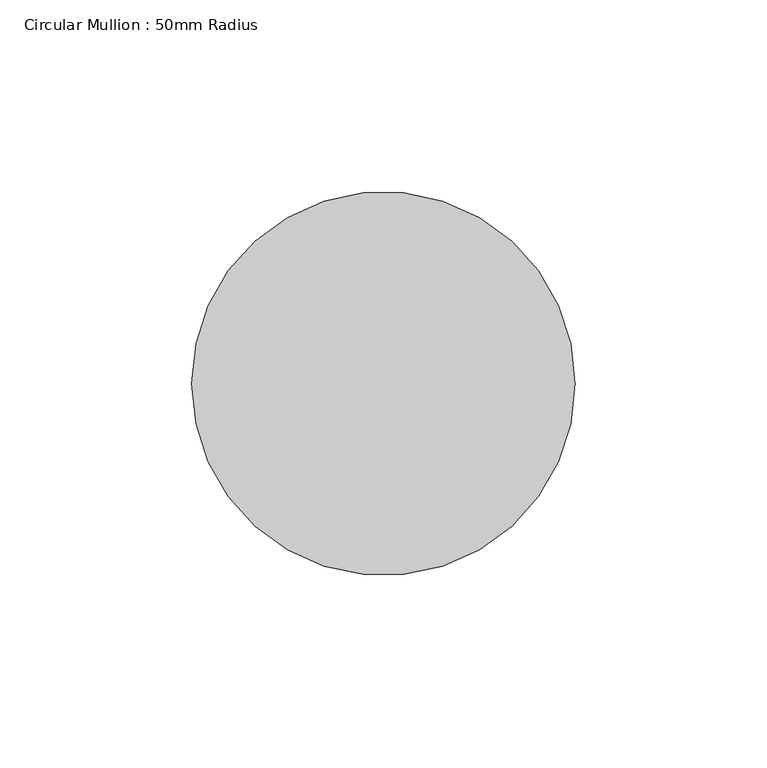
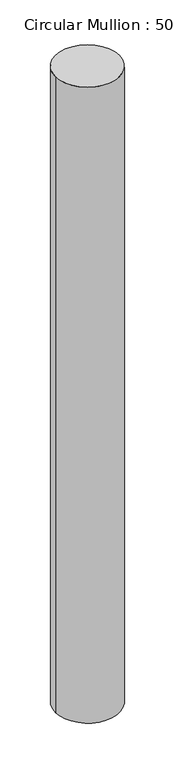
"""IFC4 building model written with IfcOpenShell, lengths in millimetres: member geometry, Circular Mullion : 50mm Radius."""

from ifc_helpers import new_model, si_unit, point, frame, origin, origin_2d, place, context, project, spatial, circle_curve, trimmed, segment, composite_curve, outline, extrude, source, transform, mapped, element, save


def circular_mullion_50mm_radius_3da29676(model_context):
    return source(origin(), model_context, "Body", "SweptSolid", [
        extrude(outline(composite_curve([segment(trimmed(circle_curve(origin_2d(), 50.0), [point((50.0, 0.0))], [point((-50.0, 0.0))], False, "CARTESIAN"), True, "CONTINUOUS"), segment(trimmed(circle_curve(origin_2d(), 50.0), [point((-50.0, 0.0))], [point((50.0, 0.0))], False, "CARTESIAN"), True, "CONTINUOUS")], self_intersect=False)), frame((0.0, 0.0, -1047.9365196), z_axis=(0.0, 0.0, 1.0), x_axis=(1.0, 0.0, 0.0)), (0.0, 0.0, 1.0), 1047.9365196),
    ])


if __name__ == "__main__":
    model = new_model("IFC4")
    model_context = context("Model", 3, world=origin())
    ifc_project = project(units=[si_unit("LENGTHUNIT", "METRE", prefix="MILLI")], contexts=[model_context])
    site = spatial("IfcSite", under=ifc_project)
    building = spatial("IfcBuilding", under=site)
    placement = place(None, origin())
    circular_mullion_50mm_radius_shape = circular_mullion_50mm_radius_3da29676(model_context)
    element("IfcMember", 1, ObjectType="Circular Mullion : 50mm Radius", at=placement, inside=building, context=model_context, shape_type="MappedRepresentation", body=[
        mapped(circular_mullion_50mm_radius_shape, transform((0.0, 0.0, 0.0), x_axis=(1.0, 0.0, 0.0), y_axis=(0.0, 1.0, 0.0), z_axis=(0.0, 0.0, 1.0))),
    ])
    save(model, "model.ifc")

# Revit data of these elements
# Type "Circular Mullion : 50mm Radius"
#   built-in parameter 1007350 = 0.164042 (stored number, unit not read)
# Element 1 (IfcMember, "Circular Mullion : 50mm Radius")
#   Materials on its faces: "Aluminium"
# Materials
#   "Aluminium": class "Metal", colour RGB 247 247 247, transparency 0, Description = "Aluminium 6061", Cost = 0
